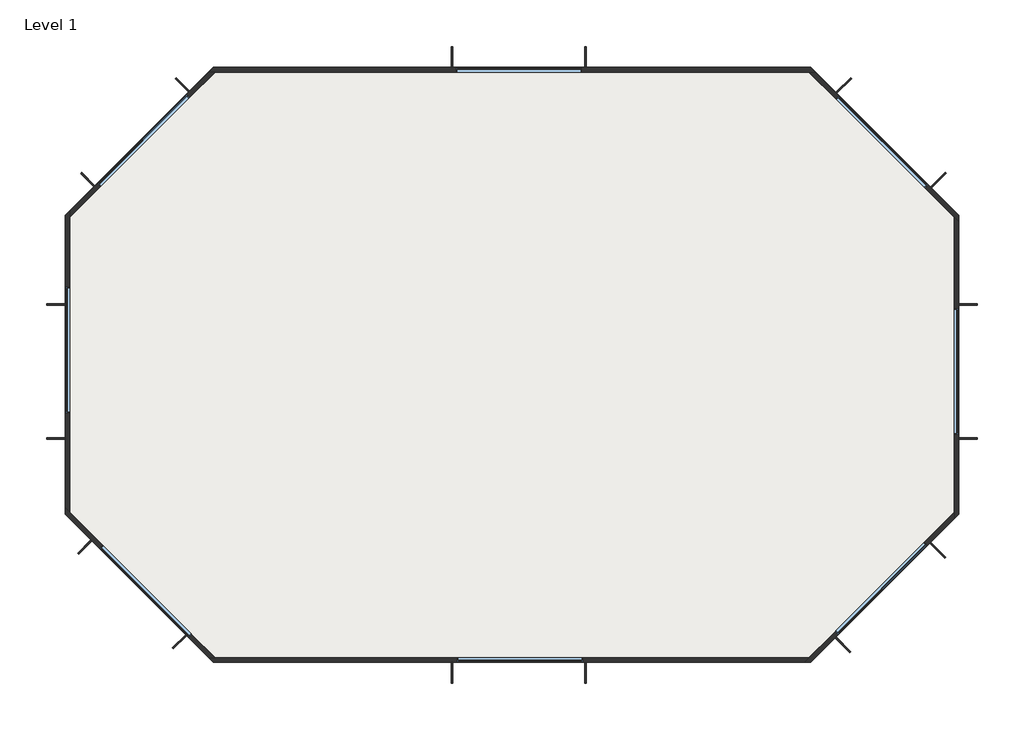
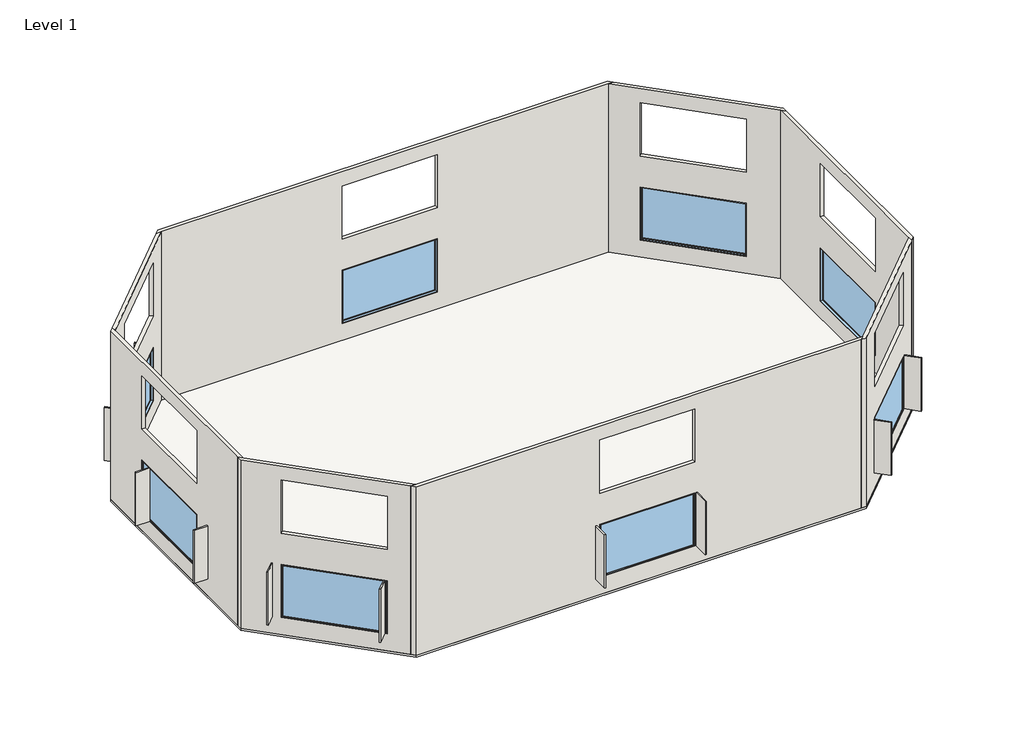
# One storey: 24 walls, 8 windows, 1 slab.
"""IFC4 building model written with IfcOpenShell, lengths in millimetres."""

import ifcopenshell
import ifcopenshell.guid

model = None  # the IFC model being written
_history = None  # IfcOwnerHistory: only IFC2X3 demands one
_inside = {}  # id of a spatial element -> (the spatial element, [elements in it])
_under = {}  # id of a project, library or spatial element -> (it, [spatial elements below it])
_declared = {}  # id of a project -> (the project, [libraries it declares])
_typed = {}  # id of a type object -> (the type object, [elements of that type])
_made_of = {}  # id of a material, layer set ... -> (it, [elements and type objects made of it])


def new_model(schema):
    """Start an empty IFC model of exactly this schema.

    Asked for "IFC4X3", IfcOpenShell would pick the latest addendum, in which some entities
    have other attributes; the version numbers below select the first issue.
    IFC2X3 requires an IfcOwnerHistory on every rooted entity: one is made here for all.
    """
    global model, _history
    if schema == "IFC4X3":
        model = ifcopenshell.file(schema_version=(4, 3, 0, 0))
    else:
        model = ifcopenshell.file(schema=schema)
    _inside.clear()
    _under.clear()
    _declared.clear()
    _typed.clear()
    _made_of.clear()
    _history = None
    if model.schema == "IFC2X3":
        org = make("IfcOrganization", Name="unknown")
        user = make(
            "IfcPersonAndOrganization",
            ThePerson=make("IfcPerson", FamilyName="unknown"),
            TheOrganization=org,
        )
        app = make(
            "IfcApplication",
            ApplicationDeveloper=org,
            Version="unknown",
            ApplicationFullName="unknown",
            ApplicationIdentifier="unknown",
        )
        _history = make(
            "IfcOwnerHistory",
            OwningUser=user,
            OwningApplication=app,
            ChangeAction="ADDED",
            CreationDate=0,
        )
    return model


def make(cls, **values):
    """One entity of the class cls with the attributes given. An attribute that is None is left unset."""
    return model.create_entity(
        cls, **{name: value for name, value in values.items() if value is not None}
    )


def rooted(cls, **values):
    """An entity with a GlobalId (a new one), such as an element, a storey or a relation."""
    return make(cls, GlobalId=ifcopenshell.guid.new(), OwnerHistory=_history, **values)


def si_unit(unit_type, name, prefix=None):
    """IfcSIUnit, for example si_unit("LENGTHUNIT", "METRE", prefix="MILLI")."""
    return make("IfcSIUnit", UnitType=unit_type, Prefix=prefix, Name=name)


def assignment(units):
    """IfcUnitAssignment: the units of a project."""
    return None if units is None else make("IfcUnitAssignment", Units=units)


def point(xyz):
    """IfcCartesianPoint."""
    return None if xyz is None else make("IfcCartesianPoint", Coordinates=xyz)


def direction(xyz):
    """IfcDirection."""
    return None if xyz is None else make("IfcDirection", DirectionRatios=xyz)


def frame(location, z_axis=None, x_axis=None):
    """IfcAxis2Placement3D, a coordinate frame: its origin and axes. An axis left out is left unset."""
    return make(
        "IfcAxis2Placement3D",
        Location=point(location),
        Axis=direction(z_axis),
        RefDirection=direction(x_axis),
    )


def origin():
    """The frame at (0, 0, 0) with its axes left unset."""
    return frame((0.0, 0.0, 0.0))


def place(relative_to, where):
    """IfcLocalPlacement: puts the frame where relative to a parent placement (None: the world)."""
    return make(
        "IfcLocalPlacement", PlacementRelTo=relative_to, RelativePlacement=where
    )


def context(
    kind, dimensions, precision=None, world=None, true_north=None, identifier=None
):
    """IfcGeometricRepresentationContext, for example the 3D "Model" context."""
    return make(
        "IfcGeometricRepresentationContext",
        ContextIdentifier=identifier,
        ContextType=kind,
        CoordinateSpaceDimension=dimensions,
        Precision=precision,
        WorldCoordinateSystem=world,
        TrueNorth=true_north,
    )


def project(units=None, contexts=None):
    """IfcProject with its units and contexts."""
    return rooted(
        "IfcProject",
        Name="project",
        RepresentationContexts=contexts,
        UnitsInContext=assignment(units),
    )


def spatial(cls, under=None, at=None, **own):
    """A site, building, storey or space (cls), placed at a placement, below another one or the project."""
    s = rooted(cls, ObjectPlacement=at, **own)
    if under is not None:
        _under.setdefault(under.id(), (under, []))[1].append(s)
    return s


def polyline(points):
    """IfcPolyline through the points."""
    return make("IfcPolyline", Points=[point(p) for p in points])


def outline(outer, holes=None, kind="AREA"):
    """IfcArbitraryClosedProfileDef: a profile drawn as a closed curve; with holes, ...WithVoids."""
    if holes is None:
        return make("IfcArbitraryClosedProfileDef", ProfileType=kind, OuterCurve=outer)
    return make(
        "IfcArbitraryProfileDefWithVoids",
        ProfileType=kind,
        OuterCurve=outer,
        InnerCurves=holes,
    )


def extrude(swept, where, along, depth):
    """IfcExtrudedAreaSolid: the profile swept, set in the frame where, extruded along a direction by depth."""
    return make(
        "IfcExtrudedAreaSolid",
        SweptArea=swept,
        Position=where,
        ExtrudedDirection=direction(along),
        Depth=depth,
    )


def faces_of(points, faces, orient=None, outer=None):
    """IfcFace entities. A face is a list of loops; a loop is a list of indices into points, from 0.

    orient and outer hold one flag for each loop. By default every Orientation is true, the
    first loop of a face is its IfcFaceOuterBound and the others are IfcFaceBound.
    """
    made = []
    for i, loops in enumerate(faces):
        bounds = []
        for j, loop in enumerate(loops):
            is_outer = j == 0 if outer is None else outer[i][j]
            bounds.append(
                make(
                    "IfcFaceOuterBound" if is_outer else "IfcFaceBound",
                    Bound=make("IfcPolyLoop", Polygon=[points[k] for k in loop]),
                    Orientation=True if orient is None else orient[i][j],
                )
            )
        made.append(make("IfcFace", Bounds=bounds))
    return made


def faceted_brep(points, faces, orient=None, outer=None, voids=None):
    """IfcFacetedBrep: a solid bounded by flat faces; with voids (closed shells), ...WithVoids."""
    shared = [point(p) for p in points]
    hull = make("IfcClosedShell", CfsFaces=faces_of(shared, faces, orient, outer))
    if voids is None:
        return make("IfcFacetedBrep", Outer=hull)
    return make(
        "IfcFacetedBrepWithVoids",
        Outer=hull,
        Voids=[
            make(cls, CfsFaces=faces_of(shared, fs, o, b)) for cls, fs, o, b in voids
        ],
    )


def shape(context_of_items, identifier, shape_type, items):
    """IfcShapeRepresentation: the items that make up one representation, for example the "Body"."""
    return make(
        "IfcShapeRepresentation",
        ContextOfItems=context_of_items,
        RepresentationIdentifier=identifier,
        RepresentationType=shape_type,
        Items=items,
    )


def source(mapping_origin, context_of_items, identifier, shape_type, items):
    """IfcRepresentationMap: a shape defined once, which mapped items show again and again."""
    return make(
        "IfcRepresentationMap",
        MappingOrigin=mapping_origin,
        MappedRepresentation=shape(context_of_items, identifier, shape_type, items),
    )


def transform(
    local_origin,
    x_axis=None,
    y_axis=None,
    z_axis=None,
    scale=None,
    scale2=None,
    scale3=None,
    uniform=True,
):
    """IfcCartesianTransformationOperator3D, or its non-uniform kind. x_axis, y_axis, z_axis: its Axis1, 2, 3."""
    if uniform:
        return make(
            "IfcCartesianTransformationOperator3D",
            Axis1=direction(x_axis),
            Axis2=direction(y_axis),
            LocalOrigin=point(local_origin),
            Scale=scale,
            Axis3=direction(z_axis),
        )
    return make(
        "IfcCartesianTransformationOperator3DnonUniform",
        Axis1=direction(x_axis),
        Axis2=direction(y_axis),
        LocalOrigin=point(local_origin),
        Scale=scale,
        Axis3=direction(z_axis),
        Scale2=scale2,
        Scale3=scale3,
    )


def mapped(mapping_source, mapping_target):
    """IfcMappedItem: shows the shape of a source again, moved by a transform."""
    return make(
        "IfcMappedItem", MappingSource=mapping_source, MappingTarget=mapping_target
    )


def made_of(thing, what):
    """Note that an element or type object is made of a material, layer set ...; save() writes the relation."""
    if what is not None:
        _made_of.setdefault(what.id(), (what, []))[1].append(thing)
    return thing


def element(
    cls,
    number,
    at=None,
    inside=None,
    cuts=None,
    type_object=None,
    material=None,
    context=None,
    identifier="Body",
    shape_type=None,
    held_by="IfcProductDefinitionShape",
    body=None,
    shapes=None,
    **own,
):
    """One element of the class cls, such as IfcWall. Its Tag is "e" and its number.

    at: its placement. inside: the storey or other place that contains it. cuts: it is an
    opening in that element (IfcRelVoidsElement). A single representation is given by context,
    identifier, shape_type and body (its items); several are given by shapes. held_by: the class
    of the entity that holds the representations. save() writes the other relations.
    """
    e = rooted(cls, Tag="e%d" % number, ObjectPlacement=at, **own)
    if body is not None:
        shapes = [shape(context, identifier, shape_type, body)]
    if shapes is not None:
        e.Representation = make(held_by, Representations=shapes)
    if inside is not None:
        _inside.setdefault(inside.id(), (inside, []))[1].append(e)
    if cuts is not None:
        rooted(
            "IfcRelVoidsElement", RelatingBuildingElement=cuts, RelatedOpeningElement=e
        )
    if type_object is not None:
        _typed.setdefault(type_object.id(), (type_object, []))[1].append(e)
    return made_of(e, material)


def aggregate(whole, parts):
    """IfcRelAggregates: a whole, such as a stair, and the parts it consists of."""
    return rooted("IfcRelAggregates", RelatingObject=whole, RelatedObjects=parts)


def save(model, path):
    """Write the relations noted so far, then the file.

    IfcRelAggregates (storeys below a building ...), IfcRelContainedInSpatialStructure (elements
    in a storey), IfcRelDefinesByType, IfcRelAssociatesMaterial and IfcRelDeclares: one each for
    every whole, place, type object, material and project.
    """
    for whole, parts in _under.values():
        aggregate(whole, parts)
    for where, things in _inside.values():
        rooted(
            "IfcRelContainedInSpatialStructure",
            RelatedElements=things,
            RelatingStructure=where,
        )
    for kind, things in _typed.values():
        rooted("IfcRelDefinesByType", RelatedObjects=things, RelatingType=kind)
    for what, things in _made_of.values():
        rooted("IfcRelAssociatesMaterial", RelatedObjects=things, RelatingMaterial=what)
    for by, libraries in _declared.values():
        rooted("IfcRelDeclares", RelatingContext=by, RelatedDefinitions=libraries)
    model.write(path)


def m_fixed_2500x_4228mm_fd5e51e7(model_context):
    return source(origin(), model_context, "Body", "SweptSolid", [
        extrude(outline(polyline([(-2050.8, 54.2), (2050.8, 54.2), (2050.8, 42.2), (-2050.8, 42.2), (-2050.8, 54.2)])), frame((0.0, 0.0, 368.0), z_axis=(0.0, 0.0, 1.0), x_axis=(1.0, 0.0, 0.0)), (0.0, 0.0, 1.0), 2374.0),
        extrude(outline(polyline([(2786.0, -2094.8), (324.0, -2094.8), (324.0, 2094.8), (2786.0, 2094.8), (2786.0, -2094.8)]), holes=[polyline([(2742.0, -2050.8), (2742.0, 2050.8), (368.0, 2050.8), (368.0, -2050.8), (2742.0, -2050.8)])]), frame((0.0, 26.2, 0.0), z_axis=(0.0, 1.0, 0.0), x_axis=(0.0, 0.0, 1.0)), (0.0, 0.0, 1.0), 44.0),
        extrude(outline(polyline([(2805.0, -2113.8), (305.0, -2113.8), (305.0, 2113.8), (2805.0, 2113.8), (2805.0, -2113.8)]), holes=[polyline([(2786.0, -2094.8), (2786.0, 2094.8), (324.0, 2094.8), (324.0, -2094.8), (2786.0, -2094.8)])]), frame((0.0, 26.2, 0.0), z_axis=(0.0, 1.0, 0.0), x_axis=(0.0, 0.0, 1.0)), (0.0, 0.0, 1.0), 63.0),
        extrude(outline(polyline([(2805.0, -2113.8), (305.0, -2113.8), (305.0, 2113.8), (2805.0, 2113.8), (2805.0, -2113.8)]), holes=[polyline([(2773.0, -2081.8), (2773.0, 2081.8), (337.0, 2081.8), (337.0, -2081.8), (2773.0, -2081.8)])]), frame((0.0, -63.2, 0.0), z_axis=(0.0, 1.0, 0.0), x_axis=(0.0, 0.0, 1.0)), (0.0, 0.0, 1.0), 89.4),
    ])


model = new_model("IFC4")

# Units and contexts
model_context = context("Model", 3, world=origin())
ifc_project = project(units=[si_unit("LENGTHUNIT", "METRE", prefix="MILLI")], contexts=[model_context])

# Site, building, storey
site = spatial("IfcSite", under=ifc_project)
building = spatial("IfcBuilding", under=site)
storey = spatial("IfcBuildingStorey", under=building, Name="Level 1", Elevation=0.0)

# Slab
placement = place(None, origin())
element("IfcSlab", 1, ObjectType="Generic Floor - 100mm", at=placement, inside=storey, context=model_context, shape_type="SweptSolid", body=[
    extrude(outline(polyline([(10639.2142415, 11296.9802217), (30639.2142415, 11296.9802217), (35588.9617098, 6347.2327534), (35588.9617098, -3652.7672466), (30639.2142415, -8602.5147149), (10639.2142415, -8602.5147149), (5689.4667732, -3652.7672466), (5689.4667732, 6347.2327534), (10639.2142415, 11296.9802217)])), frame((0.0, 0.0, -100.0), z_axis=(0.0, 0.0, 1.0), x_axis=(1.0, 0.0, 0.0)), (0.0, 0.0, 1.0), 100.0),
])

# Walls
element("IfcWall", 2, ObjectType="Generic - 152.4mm", at=placement, inside=storey, context=model_context, shape_type="Brep", body=[
    faceted_brep([(10486.8142415, 11144.5802217, 0.0), (10702.3403884, 11144.5802217, 0.0), (30576.0880946, 11144.5802217, 0.0), (30791.6142415, 11144.5802217, 0.0), (30791.6142415, 11144.5802217, 7924.8), (30576.0880946, 11144.5802217, 7924.8), (10702.3403884, 11144.5802217, 7924.8), (10486.8142415, 11144.5802217, 7924.8), (18752.7836697, 11144.5802217, 4762.4), (18752.7836697, 11144.5802217, 7262.4), (22980.3836697, 11144.5802217, 7262.4), (22980.3836697, 11144.5802217, 4762.4), (18752.7836697, 11144.5802217, 800.0), (18752.7836697, 11144.5802217, 3300.0), (22980.3836697, 11144.5802217, 3300.0), (22980.3836697, 11144.5802217, 800.0), (10639.2142415, 11296.9802217, 0.0), (10639.2142415, 11296.9802217, 7924.8), (30639.2142415, 11296.9802217, 7924.8), (30639.2142415, 11296.9802217, 0.0), (18752.7836697, 11296.9802217, 4762.4), (22980.3836697, 11296.9802217, 4762.4), (22980.3836697, 11296.9802217, 7262.4), (18752.7836697, 11296.9802217, 7262.4), (18752.7836697, 11296.9802217, 800.0), (22980.3836697, 11296.9802217, 800.0), (22980.3836697, 11296.9802217, 3300.0), (18752.7836697, 11296.9802217, 3300.0)], [[[0, 1, 2, 3, 4, 5, 6, 7], [8, 9, 10, 11], [12, 13, 14, 15]], [[16, 17, 18, 19], [20, 21, 22, 23], [24, 25, 26, 27]], [[3, 2, 1, 0, 16, 19]], [[7, 6, 5, 4, 18, 17]], [[4, 3, 19, 18]], [[0, 7, 17, 16]], [[9, 8, 20, 23]], [[10, 9, 23, 22]], [[11, 10, 22, 21]], [[8, 11, 21, 20]], [[13, 12, 24, 27]], [[14, 13, 27, 26]], [[15, 14, 26, 25]], [[12, 15, 25, 24]]]),
])
element("IfcWall", 3, ObjectType="Generic - 152.4mm", at=placement, inside=storey, context=model_context, shape_type="Brep", body=[
    faceted_brep([(30576.0880946, 11144.5802217, 0.0), (35436.5617098, 6284.1066065, 0.0), (35588.9617098, 6131.7066065, 0.0), (35588.9617098, 6131.7066065, 7924.8), (35436.5617098, 6284.1066065, 7924.8), (30576.0880946, 11144.5802217, 7924.8), (31471.8841839, 10248.7841324, 4762.4), (31471.8841839, 10248.7841324, 7262.4), (34461.2488121, 7259.4195042, 7262.4), (34461.2488121, 7259.4195042, 4762.4), (31471.8841839, 10248.7841324, 800.0), (31471.8841839, 10248.7841324, 3300.0), (34461.2488121, 7259.4195042, 3300.0), (34461.2488121, 7259.4195042, 800.0), (30791.6142415, 11144.5802217, 0.0), (30791.6142415, 11144.5802217, 7924.8), (35588.9617098, 6347.2327534, 7924.8), (35588.9617098, 6347.2327534, 0.0), (31579.6472574, 10356.5472058, 4762.4), (34569.0118855, 7367.1825777, 4762.4), (34569.0118855, 7367.1825777, 7262.4), (31579.6472574, 10356.5472058, 7262.4), (31579.6472574, 10356.5472058, 800.0), (34569.0118855, 7367.1825777, 800.0), (34569.0118855, 7367.1825777, 3300.0), (31579.6472574, 10356.5472058, 3300.0)], [[[0, 1, 2, 3, 4, 5], [6, 7, 8, 9], [10, 11, 12, 13]], [[14, 15, 16, 17], [18, 19, 20, 21], [22, 23, 24, 25]], [[2, 1, 0, 14, 17]], [[5, 4, 3, 16, 15]], [[0, 5, 15, 14]], [[3, 2, 17, 16]], [[7, 6, 18, 21]], [[8, 7, 21, 20]], [[9, 8, 20, 19]], [[6, 9, 19, 18]], [[11, 10, 22, 25]], [[12, 11, 25, 24]], [[13, 12, 24, 23]], [[10, 13, 23, 22]]]),
])
element("IfcWall", 4, ObjectType="Generic - 152.4mm", at=placement, inside=storey, context=model_context, shape_type="Brep", body=[
    faceted_brep([(35436.5617098, 6284.1066065, 0.0), (35436.5617098, -3589.6410997, 0.0), (35436.5617098, -3805.1672466, 0.0), (35436.5617098, -3805.1672466, 7924.8), (35436.5617098, -3589.6410997, 7924.8), (35436.5617098, 6284.1066065, 7924.8), (35436.5617098, 3236.2401206, 4762.4), (35436.5617098, 3236.2401206, 7262.4), (35436.5617098, -991.3598794, 7262.4), (35436.5617098, -991.3598794, 4762.4), (35436.5617098, 3236.2401206, 800.0), (35436.5617098, 3236.2401206, 3300.0), (35436.5617098, -991.3598794, 3300.0), (35436.5617098, -991.3598794, 800.0), (35588.9617098, 6131.7066065, 0.0), (35588.9617098, 6131.7066065, 7924.8), (35588.9617098, -3652.7672466, 7924.8), (35588.9617098, -3652.7672466, 0.0), (35588.9617098, 3236.2401206, 4762.4), (35588.9617098, -991.3598794, 4762.4), (35588.9617098, -991.3598794, 7262.4), (35588.9617098, 3236.2401206, 7262.4), (35588.9617098, 3236.2401206, 800.0), (35588.9617098, -991.3598794, 800.0), (35588.9617098, -991.3598794, 3300.0), (35588.9617098, 3236.2401206, 3300.0)], [[[0, 1, 2, 3, 4, 5], [6, 7, 8, 9], [10, 11, 12, 13]], [[14, 15, 16, 17], [18, 19, 20, 21], [22, 23, 24, 25]], [[2, 1, 0, 14, 17]], [[5, 4, 3, 16, 15]], [[0, 5, 15, 14]], [[3, 2, 17, 16]], [[7, 6, 18, 21]], [[8, 7, 21, 20]], [[9, 8, 20, 19]], [[6, 9, 19, 18]], [[11, 10, 22, 25]], [[12, 11, 25, 24]], [[13, 12, 24, 23]], [[10, 13, 23, 22]]]),
])
element("IfcWall", 5, ObjectType="Generic - 152.4mm", at=placement, inside=storey, context=model_context, shape_type="Brep", body=[
    faceted_brep([(35436.5617098, -3589.6410997, 0.0), (30576.0880946, -8450.1147149, 0.0), (30423.6880946, -8602.5147149, 0.0), (30423.6880946, -8602.5147149, 7924.8), (30576.0880946, -8450.1147149, 7924.8), (35436.5617098, -3589.6410997, 7924.8), (34437.5479697, -4588.6548399, 4762.4), (34437.5479697, -4588.6548399, 7262.4), (31448.1833416, -7578.019468, 7262.4), (31448.1833416, -7578.019468, 4762.4), (34437.5479697, -4588.6548399, 800.0), (34437.5479697, -4588.6548399, 3300.0), (31448.1833416, -7578.019468, 3300.0), (31448.1833416, -7578.019468, 800.0), (30639.2142415, -8602.5147149, 0.0), (35436.5617098, -3805.1672466, 0.0), (35436.5617098, -3805.1672466, 7924.8), (30639.2142415, -8602.5147149, 7924.8), (34545.3110432, -4696.4179133, 7262.4), (34545.3110432, -4696.4179133, 4762.4), (31555.946415, -7685.7825415, 4762.4), (31555.946415, -7685.7825415, 7262.4), (34545.3110432, -4696.4179133, 3300.0), (34545.3110432, -4696.4179133, 800.0), (31555.946415, -7685.7825415, 800.0), (31555.946415, -7685.7825415, 3300.0)], [[[0, 1, 2, 3, 4, 5], [6, 7, 8, 9], [10, 11, 12, 13]], [[14, 15, 16, 17], [18, 19, 20, 21], [22, 23, 24, 25]], [[2, 1, 0, 15, 14]], [[5, 4, 3, 17, 16]], [[0, 5, 16, 15]], [[3, 2, 14, 17]], [[6, 19, 18, 7]], [[7, 18, 21, 8]], [[8, 21, 20, 9]], [[19, 6, 9, 20]], [[11, 10, 23, 22]], [[12, 11, 22, 25]], [[13, 12, 25, 24]], [[10, 13, 24, 23]]]),
])
element("IfcWall", 6, ObjectType="Generic - 152.4mm", at=placement, inside=storey, context=model_context, shape_type="Brep", body=[
    faceted_brep([(30576.0880946, -8450.1147149, 0.0), (10702.3403884, -8450.1147149, 0.0), (10486.8142415, -8450.1147149, 0.0), (10486.8142415, -8450.1147149, 7924.8), (10702.3403884, -8450.1147149, 7924.8), (30576.0880946, -8450.1147149, 7924.8), (23020.9791073, -8450.1147149, 4762.4), (23020.9791073, -8450.1147149, 7262.4), (18793.3791073, -8450.1147149, 7262.4), (18793.3791073, -8450.1147149, 4762.4), (23020.9791073, -8450.1147149, 800.0), (23020.9791073, -8450.1147149, 3300.0), (18793.3791073, -8450.1147149, 3300.0), (18793.3791073, -8450.1147149, 800.0), (30423.6880946, -8602.5147149, 0.0), (30423.6880946, -8602.5147149, 7924.8), (10639.2142415, -8602.5147149, 7924.8), (10639.2142415, -8602.5147149, 0.0), (23020.9791073, -8602.5147149, 4762.4), (18793.3791073, -8602.5147149, 4762.4), (18793.3791073, -8602.5147149, 7262.4), (23020.9791073, -8602.5147149, 7262.4), (23020.9791073, -8602.5147149, 800.0), (18793.3791073, -8602.5147149, 800.0), (18793.3791073, -8602.5147149, 3300.0), (23020.9791073, -8602.5147149, 3300.0)], [[[0, 1, 2, 3, 4, 5], [6, 7, 8, 9], [10, 11, 12, 13]], [[14, 15, 16, 17], [18, 19, 20, 21], [22, 23, 24, 25]], [[2, 1, 0, 14, 17]], [[5, 4, 3, 16, 15]], [[0, 5, 15, 14]], [[3, 2, 17, 16]], [[7, 6, 18, 21]], [[8, 7, 21, 20]], [[9, 8, 20, 19]], [[6, 9, 19, 18]], [[11, 10, 22, 25]], [[12, 11, 25, 24]], [[13, 12, 24, 23]], [[10, 13, 23, 22]]]),
])
element("IfcWall", 7, ObjectType="Generic - 152.4mm", at=placement, inside=storey, context=model_context, shape_type="Brep", body=[
    faceted_brep([(10702.3403884, -8450.1147149, 0.0), (5841.8667732, -3589.6410997, 0.0), (5689.4667732, -3437.2410997, 0.0), (5689.4667732, -3437.2410997, 7924.8), (5841.8667732, -3589.6410997, 7924.8), (10702.3403884, -8450.1147149, 7924.8), (9927.9208562, -7675.6951827, 4762.4), (9927.9208562, -7675.6951827, 7262.4), (6938.556228, -4686.3305545, 7262.4), (6938.556228, -4686.3305545, 4762.4), (9927.9208562, -7675.6951827, 800.0), (9927.9208562, -7675.6951827, 3300.0), (6938.556228, -4686.3305545, 3300.0), (6938.556228, -4686.3305545, 800.0), (10486.8142415, -8450.1147149, 0.0), (10486.8142415, -8450.1147149, 7924.8), (5689.4667732, -3652.7672466, 7924.8), (5689.4667732, -3652.7672466, 0.0), (9820.1577827, -7783.4582561, 4762.4), (6830.7931546, -4794.093628, 4762.4), (6830.7931546, -4794.093628, 7262.4), (9820.1577827, -7783.4582561, 7262.4), (9820.1577827, -7783.4582561, 800.0), (6830.7931546, -4794.093628, 800.0), (6830.7931546, -4794.093628, 3300.0), (9820.1577827, -7783.4582561, 3300.0)], [[[0, 1, 2, 3, 4, 5], [6, 7, 8, 9], [10, 11, 12, 13]], [[14, 15, 16, 17], [18, 19, 20, 21], [22, 23, 24, 25]], [[2, 1, 0, 14, 17]], [[5, 4, 3, 16, 15]], [[0, 5, 15, 14]], [[3, 2, 17, 16]], [[7, 6, 18, 21]], [[8, 7, 21, 20]], [[9, 8, 20, 19]], [[6, 9, 19, 18]], [[11, 10, 22, 25]], [[12, 11, 25, 24]], [[13, 12, 24, 23]], [[10, 13, 23, 22]]]),
])
element("IfcWall", 8, ObjectType="Generic - 152.4mm", at=placement, inside=storey, context=model_context, shape_type="Brep", body=[
    faceted_brep([(5841.8667732, -3589.6410997, 0.0), (5841.8667732, 6284.1066065, 0.0), (5841.8667732, 6499.6327534, 0.0), (5841.8667732, 6499.6327534, 7924.8), (5841.8667732, 6284.1066065, 7924.8), (5841.8667732, -3589.6410997, 7924.8), (5841.8667732, -270.991266, 4762.4), (5841.8667732, -270.991266, 7262.4), (5841.8667732, 3956.608734, 7262.4), (5841.8667732, 3956.608734, 4762.4), (5841.8667732, -270.991266, 800.0), (5841.8667732, -270.991266, 3300.0), (5841.8667732, 3956.608734, 3300.0), (5841.8667732, 3956.608734, 800.0), (5689.4667732, -3437.2410997, 0.0), (5689.4667732, -3437.2410997, 7924.8), (5689.4667732, 6347.2327534, 7924.8), (5689.4667732, 6347.2327534, 0.0), (5689.4667732, -270.991266, 4762.4), (5689.4667732, 3956.608734, 4762.4), (5689.4667732, 3956.608734, 7262.4), (5689.4667732, -270.991266, 7262.4), (5689.4667732, -270.991266, 800.0), (5689.4667732, 3956.608734, 800.0), (5689.4667732, 3956.608734, 3300.0), (5689.4667732, -270.991266, 3300.0)], [[[0, 1, 2, 3, 4, 5], [6, 7, 8, 9], [10, 11, 12, 13]], [[14, 15, 16, 17], [18, 19, 20, 21], [22, 23, 24, 25]], [[2, 1, 0, 14, 17]], [[5, 4, 3, 16, 15]], [[0, 5, 15, 14]], [[3, 2, 17, 16]], [[7, 6, 18, 21]], [[8, 7, 21, 20]], [[9, 8, 20, 19]], [[6, 9, 19, 18]], [[11, 10, 22, 25]], [[12, 11, 25, 24]], [[13, 12, 24, 23]], [[10, 13, 23, 22]]]),
])
element("IfcWall", 9, ObjectType="Generic - 152.4mm", at=placement, inside=storey, context=model_context, shape_type="Brep", body=[
    faceted_brep([(5841.8667732, 6284.1066065, 0.0), (10702.3403884, 11144.5802217, 0.0), (10702.3403884, 11144.5802217, 7924.8), (5841.8667732, 6284.1066065, 7924.8), (6863.3827465, 7305.6225798, 4762.4), (6863.3827465, 7305.6225798, 7262.4), (9852.7473747, 10294.9872079, 7262.4), (9852.7473747, 10294.9872079, 4762.4), (6863.3827465, 7305.6225798, 800.0), (6863.3827465, 7305.6225798, 3300.0), (9852.7473747, 10294.9872079, 3300.0), (9852.7473747, 10294.9872079, 800.0), (5841.8667732, 6499.6327534, 0.0), (5841.8667732, 6499.6327534, 7924.8), (10486.8142415, 11144.5802217, 7924.8), (10486.8142415, 11144.5802217, 0.0), (6755.6196731, 7413.3856532, 4762.4), (9744.9843012, 10402.7502814, 4762.4), (9744.9843012, 10402.7502814, 7262.4), (6755.6196731, 7413.3856532, 7262.4), (6755.6196731, 7413.3856532, 800.0), (9744.9843012, 10402.7502814, 800.0), (9744.9843012, 10402.7502814, 3300.0), (6755.6196731, 7413.3856532, 3300.0)], [[[0, 1, 2, 3], [4, 5, 6, 7], [8, 9, 10, 11]], [[12, 13, 14, 15], [16, 17, 18, 19], [20, 21, 22, 23]], [[1, 0, 12, 15]], [[3, 2, 14, 13]], [[0, 3, 13, 12]], [[2, 1, 15, 14]], [[5, 4, 16, 19]], [[6, 5, 19, 18]], [[7, 6, 18, 17]], [[4, 7, 17, 16]], [[9, 8, 20, 23]], [[10, 9, 23, 22]], [[11, 10, 22, 21]], [[8, 11, 21, 20]]]),
])
element("IfcWall", 10, ObjectType="Generic - Shading", at=placement, inside=storey, context=model_context, shape_type="SweptSolid", body=[
    extrude(outline(polyline([(18602.7836697, -9302.5147149), (18602.7836697, -8602.5147149), (18652.7836697, -8602.5147149), (18652.7836697, -9302.5147149), (18602.7836697, -9302.5147149)])), frame((0.0, 0.0, 800.0), z_axis=(0.0, 0.0, 1.0), x_axis=(1.0, 0.0, 0.0)), (0.0, 0.0, 1.0), 2500.0),
])
element("IfcWall", 11, ObjectType="Generic - Shading", at=placement, inside=storey, context=model_context, shape_type="SweptSolid", body=[
    extrude(outline(polyline([(23080.3836697, -9302.5147149), (23080.3836697, -8602.5147149), (23130.3836697, -8602.5147149), (23130.3836697, -9302.5147149), (23080.3836697, -9302.5147149)])), frame((0.0, 0.0, 800.0), z_axis=(0.0, 0.0, 1.0), x_axis=(1.0, 0.0, 0.0)), (0.0, 0.0, 1.0), 2500.0),
])
element("IfcWall", 12, ObjectType="Generic - Shading", at=placement, inside=storey, context=model_context, shape_type="SweptSolid", body=[
    extrude(outline(polyline([(18652.7836697, 11996.9802217), (18652.7836697, 11296.9802217), (18602.7836697, 11296.9802217), (18602.7836697, 11996.9802217), (18652.7836697, 11996.9802217)])), frame((0.0, 0.0, 800.0), z_axis=(0.0, 0.0, 1.0), x_axis=(1.0, 0.0, 0.0)), (0.0, 0.0, 1.0), 2500.0),
])
element("IfcWall", 13, ObjectType="Generic - Shading", at=placement, inside=storey, context=model_context, shape_type="SweptSolid", body=[
    extrude(outline(polyline([(23130.3836697, 11996.9802217), (23130.3836697, 11296.9802217), (23080.3836697, 11296.9802217), (23080.3836697, 11996.9802217), (23130.3836697, 11996.9802217)])), frame((0.0, 0.0, 800.0), z_axis=(0.0, 0.0, 1.0), x_axis=(1.0, 0.0, 0.0)), (0.0, 0.0, 1.0), 2500.0),
])
element("IfcWall", 14, ObjectType="Generic - Shading", at=placement, inside=storey, context=model_context, shape_type="SweptSolid", body=[
    extrude(outline(polyline([(32003.1901519, 10922.602081), (31508.391267, 10427.8031962), (31473.035928, 10463.1585352), (31967.8348129, 10957.9574201), (32003.1901519, 10922.602081)])), frame((0.0, 0.0, 800.0), z_axis=(0.0, 0.0, 1.0), x_axis=(1.0, 0.0, 0.0)), (0.0, 0.0, 1.0), 2500.0),
])
element("IfcWall", 15, ObjectType="Generic - Shading", at=placement, inside=storey, context=model_context, shape_type="SweptSolid", body=[
    extrude(outline(polyline([(35169.8767876, 7755.9154454), (34675.0779027, 7261.1165605), (34639.7225636, 7296.4718995), (35134.5214485, 7791.2707844), (35169.8767876, 7755.9154454)])), frame((0.0, 0.0, 800.0), z_axis=(0.0, 0.0, 1.0), x_axis=(1.0, 0.0, 0.0)), (0.0, 0.0, 1.0), 2500.0),
])
element("IfcWall", 16, ObjectType="Generic - Shading", at=placement, inside=storey, context=model_context, shape_type="SweptSolid", body=[
    extrude(outline(polyline([(31944.1339705, -8287.1927558), (31449.3350856, -7792.3938709), (31484.6904247, -7757.0385318), (31979.4893096, -8251.8374167), (31944.1339705, -8287.1927558)])), frame((0.0, 0.0, 800.0), z_axis=(0.0, 0.0, 1.0), x_axis=(1.0, 0.0, 0.0)), (0.0, 0.0, 1.0), 2500.0),
])
element("IfcWall", 17, ObjectType="Generic - Shading", at=placement, inside=storey, context=model_context, shape_type="SweptSolid", body=[
    extrude(outline(polyline([(35110.8206062, -5120.5061201), (34616.0217213, -4625.7072352), (34651.3770603, -4590.3518961), (35146.1759452, -5085.150781), (35110.8206062, -5120.5061201)])), frame((0.0, 0.0, 800.0), z_axis=(0.0, 0.0, 1.0), x_axis=(1.0, 0.0, 0.0)), (0.0, 0.0, 1.0), 2500.0),
])
element("IfcWall", 18, ObjectType="Generic - Shading", at=placement, inside=storey, context=model_context, shape_type="SweptSolid", body=[
    extrude(outline(polyline([(9410.5024205, 10950.4548209), (9851.5956306, 10509.3616108), (9816.2402916, 10474.0062717), (9375.1470815, 10915.0994818), (9410.5024205, 10950.4548209)])), frame((0.0, 0.0, 800.0), z_axis=(0.0, 0.0, 1.0), x_axis=(1.0, 0.0, 0.0)), (0.0, 0.0, 1.0), 2500.0),
])
element("IfcWall", 19, ObjectType="Generic - Shading", at=placement, inside=storey, context=model_context, shape_type="SweptSolid", body=[
    extrude(outline(polyline([(6243.8157849, 7783.7681852), (6684.908995, 7342.6749751), (6649.5536559, 7307.319636), (6208.4604458, 7748.4128461), (6243.8157849, 7783.7681852)])), frame((0.0, 0.0, 800.0), z_axis=(0.0, 0.0, 1.0), x_axis=(1.0, 0.0, 0.0)), (0.0, 0.0, 1.0), 2500.0),
])
element("IfcWall", 20, ObjectType="Generic - Shading", at=placement, inside=storey, context=model_context, shape_type="SweptSolid", body=[
    extrude(outline(polyline([(9275.0624692, -8120.5493628), (9716.1556793, -7679.4561527), (9751.5110184, -7714.8114918), (9310.4178082, -8155.9047019), (9275.0624692, -8120.5493628)])), frame((0.0, 0.0, 800.0), z_axis=(0.0, 0.0, 1.0), x_axis=(1.0, 0.0, 0.0)), (0.0, 0.0, 1.0), 2500.0),
])
element("IfcWall", 21, ObjectType="Generic - Shading", at=placement, inside=storey, context=model_context, shape_type="SweptSolid", body=[
    extrude(outline(polyline([(6108.3758335, -4953.8627272), (6549.4690436, -4512.769517), (6584.8243827, -4548.1248561), (6143.7311726, -4989.2180662), (6108.3758335, -4953.8627272)])), frame((0.0, 0.0, 800.0), z_axis=(0.0, 0.0, 1.0), x_axis=(1.0, 0.0, 0.0)), (0.0, 0.0, 1.0), 2500.0),
])
element("IfcWall", 22, ObjectType="Generic - Shading", at=placement, inside=storey, context=model_context, shape_type="SweptSolid", body=[
    extrude(outline(polyline([(36212.7617098, -1141.3598794), (35588.9617098, -1141.3598794), (35588.9617098, -1091.3598794), (36212.7617098, -1091.3598794), (36212.7617098, -1141.3598794)])), frame((0.0, 0.0, 800.0), z_axis=(0.0, 0.0, 1.0), x_axis=(1.0, 0.0, 0.0)), (0.0, 0.0, 1.0), 2500.0),
])
element("IfcWall", 23, ObjectType="Generic - Shading", at=placement, inside=storey, context=model_context, shape_type="SweptSolid", body=[
    extrude(outline(polyline([(36212.7617098, 3336.2401206), (35588.9617098, 3336.2401206), (35588.9617098, 3386.2401206), (36212.7617098, 3386.2401206), (36212.7617098, 3336.2401206)])), frame((0.0, 0.0, 800.0), z_axis=(0.0, 0.0, 1.0), x_axis=(1.0, 0.0, 0.0)), (0.0, 0.0, 1.0), 2500.0),
])
element("IfcWall", 24, ObjectType="Generic - Shading", at=placement, inside=storey, context=model_context, shape_type="SweptSolid", body=[
    extrude(outline(polyline([(5065.6667732, -1091.3598794), (5689.4667732, -1091.3598794), (5689.4667732, -1141.3598794), (5065.6667732, -1141.3598794), (5065.6667732, -1091.3598794)])), frame((0.0, 0.0, 800.0), z_axis=(0.0, 0.0, 1.0), x_axis=(1.0, 0.0, 0.0)), (0.0, 0.0, 1.0), 2500.0),
])
element("IfcWall", 25, ObjectType="Generic - Shading", at=placement, inside=storey, context=model_context, shape_type="SweptSolid", body=[
    extrude(outline(polyline([(5065.6667732, 3386.2401206), (5689.4667732, 3386.2401206), (5689.4667732, 3336.2401206), (5065.6667732, 3336.2401206), (5065.6667732, 3386.2401206)])), frame((0.0, 0.0, 800.0), z_axis=(0.0, 0.0, 1.0), x_axis=(1.0, 0.0, 0.0)), (0.0, 0.0, 1.0), 2500.0),
])

# Windows
m_fixed_2500x_4228mm_shape = m_fixed_2500x_4228mm_fd5e51e7(model_context)
element("IfcWindow", 26, ObjectType="M_Fixed : 2500X 4228mm", at=placement, inside=storey, context=model_context, shape_type="MappedRepresentation", body=[
    mapped(m_fixed_2500x_4228mm_shape, transform((20907.1791073, -8513.3147149, 495.0), x_axis=(-1.0, 0.0, 0.0), y_axis=(0.0, -1.0, 0.0), z_axis=(0.0, 0.0, 1.0))),
])
element("IfcWindow", 27, ObjectType="M_Fixed : 2500X 4228mm", at=placement, inside=storey, context=model_context, shape_type="MappedRepresentation", body=[
    mapped(m_fixed_2500x_4228mm_shape, transform((32987.5548042, -6128.0263025, 495.0), x_axis=(-0.707106781186548, -0.7071067811865471, 0.0), y_axis=(0.7071067811865471, -0.707106781186548, 0.0), z_axis=(0.0, 0.0, 1.0))),
])
element("IfcWindow", 28, ObjectType="M_Fixed : 2500X 4228mm", at=placement, inside=storey, context=model_context, shape_type="MappedRepresentation", body=[
    mapped(m_fixed_2500x_4228mm_shape, transform((35499.7617098, 1122.4401206, 495.0), x_axis=(0.0, -1.0, 0.0), y_axis=(1.0, 0.0, 0.0), z_axis=(0.0, 0.0, 1.0))),
])
element("IfcWindow", 29, ObjectType="M_Fixed : 2500X 4228mm", at=placement, inside=storey, context=model_context, shape_type="MappedRepresentation", body=[
    mapped(m_fixed_2500x_4228mm_shape, transform((33011.2556466, 8798.7909669, 495.0), x_axis=(0.7071067811865468, -0.7071067811865483, 0.0), y_axis=(0.7071067811865483, 0.7071067811865468, 0.0), z_axis=(0.0, 0.0, 1.0))),
])
element("IfcWindow", 30, ObjectType="M_Fixed : 2500X 4228mm", at=placement, inside=storey, context=model_context, shape_type="MappedRepresentation", body=[
    mapped(m_fixed_2500x_4228mm_shape, transform((20866.5836697, 11207.7802217, 495.0), x_axis=(1.0, 0.0, 0.0), y_axis=(0.0, 1.0, 0.0), z_axis=(0.0, 0.0, 1.0))),
])
element("IfcWindow", 31, ObjectType="M_Fixed : 2500X 4228mm", at=placement, inside=storey, context=model_context, shape_type="MappedRepresentation", body=[
    mapped(m_fixed_2500x_4228mm_shape, transform((8313.375912, 8844.9940424, 495.0), x_axis=(0.7071067811865479, 0.707106781186547, 0.0), y_axis=(-0.707106781186547, 0.7071067811865479, 0.0), z_axis=(0.0, 0.0, 1.0))),
])
element("IfcWindow", 32, ObjectType="M_Fixed : 2500X 4228mm", at=placement, inside=storey, context=model_context, shape_type="MappedRepresentation", body=[
    mapped(m_fixed_2500x_4228mm_shape, transform((5778.6667732, 1842.808734, 495.0), x_axis=(0.0, 1.0, 0.0), y_axis=(-1.0, 0.0, 0.0), z_axis=(0.0, 0.0, 1.0))),
])
element("IfcWindow", 33, ObjectType="M_Fixed : 2500X 4228mm", at=placement, inside=storey, context=model_context, shape_type="MappedRepresentation", body=[
    mapped(m_fixed_2500x_4228mm_shape, transform((8388.5493935, -6225.7020172, 495.0), x_axis=(-0.707106781186546, 0.707106781186549, 0.0), y_axis=(-0.707106781186549, -0.707106781186546, 0.0), z_axis=(0.0, 0.0, 1.0))),
])

save(model, "model.ifc")

# Revit data of these elements
# Project information
#   Project Issue Date = "Issue Date"
#   Project Status = "Project Status"
#   Client Name = "Owner"
#   Project Address = "Enter address here"
#   Project Name = "Project Name"
#   Project Number = "Project Number"
# Type "Generic Floor - 100mm"
#   Function = 0
#   Layers, outside or top first: 100 mm no material (function 1)
# Type "Generic - 152.4mm"
#   Layers, outside or top first: 152.4 mm no material (function 1)
# Type "Generic - Shading"
#   Layers, outside or top first: 50 mm no material (function 1)
# Type "M_Fixed : 2500X 4228mm"
#   Type Mark = "25"
#   Height = 2500 mm
#   Default Sill Height = 305 mm
#   Width = 4227.6 mm
#   Window Inset = 19 mm
#   Frame Exterior Material = Sash
#   Frame Interior Material = Sash
#   Glass Pane Material = Glass
#   Sash = Sash
#   Wall Closure = (empty or 0)
# Element 1 (IfcSlab, "Generic Floor - 100mm")
#   built-in parameter 1001955 = 0.785398 (stored number, unit not read)
#   Height Offset From Level = 0 mm
#   Phase Created = New Construction
#   Materials on its faces: "Default Floor"
# Elements 2, 3, 4, 5, 6, 7, 8, 9 (IfcWall, "Generic - 152.4mm")
#   Top Offset = 0 mm
#   Base Offset = 0 mm
#   wall height = 7924.8 mm
#   Phase Created = New Construction
#   Base Constraint = Level 1
#   Top Constraint = Roof Level
#   Materials on its faces: "Default Wall"
# Elements 10, 11, 12, 13, 22, 23, 24, 25 (IfcWall, "Generic - Shading")
#   built-in parameter 1001111 = 800 mm
#   Top Offset = -662.4 mm
#   Base Offset = 800 mm
#   wall height = 2500 mm
#   Phase Created = New Construction
#   Base Constraint = Level 1
#   Top Constraint = Level 2
#   Materials on its faces: "Default Wall"
# Elements 14, 15, 16, 17, 18, 19, 20, 21 (IfcWall, "Generic - Shading")
#   built-in parameter 1001111 = 800 mm
#   Top Offset = -4624.8 mm
#   Base Offset = 800 mm
#   wall height = 2500 mm
#   Phase Created = New Construction
#   Base Constraint = Level 1
#   Top Constraint = Roof Level
#   Materials on its faces: "Default Wall"
# Element 26 (IfcWindow, "M_Fixed : 2500X 4228mm")
#   Mark = "38"
#   Phase Created = New Construction
#   Materials on its faces: "Sash", "Glass"
# Element 27 (IfcWindow, "M_Fixed : 2500X 4228mm")
#   Mark = "39"
#   Phase Created = New Construction
#   Materials on its faces: "Sash", "Glass"
# Element 28 (IfcWindow, "M_Fixed : 2500X 4228mm")
#   Mark = "40"
#   Phase Created = New Construction
#   Materials on its faces: "Sash", "Glass"
# Element 29 (IfcWindow, "M_Fixed : 2500X 4228mm")
#   Mark = "41"
#   Phase Created = New Construction
#   Materials on its faces: "Sash", "Glass"
# Element 30 (IfcWindow, "M_Fixed : 2500X 4228mm")
#   Mark = "42"
#   Phase Created = New Construction
#   Materials on its faces: "Sash", "Glass"
# Element 31 (IfcWindow, "M_Fixed : 2500X 4228mm")
#   Mark = "43"
#   Phase Created = New Construction
#   Materials on its faces: "Sash", "Glass"
# Element 32 (IfcWindow, "M_Fixed : 2500X 4228mm")
#   Mark = "44"
#   Phase Created = New Construction
#   Materials on its faces: "Sash", "Glass"
# Element 33 (IfcWindow, "M_Fixed : 2500X 4228mm")
#   Mark = "45"
#   Phase Created = New Construction
#   Materials on its faces: "Sash", "Glass"
# Materials
#   "Sash": class "Wood", colour RGB 136 99 55, transparency 0
#   "Glass": class "Glass", colour RGB 0 128 192, transparency 0.9, Description = "Soda Lime Glass", Cost = 0
#   "Default Floor": class "Miscellaneous", colour RGB 127 127 127, transparency 0, Cost = 0
#   "Default Wall": class "Miscellaneous", colour RGB 128 128 128, transparency 0, Cost = 0
# Room at (20073.113, 2003.303) mm, phase "New Construction", upper level "Level 1", upper offset 3962.4 mm, lower offset 0 mm
#   Number = "11"
#   Name = "Room"
